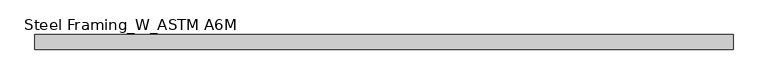
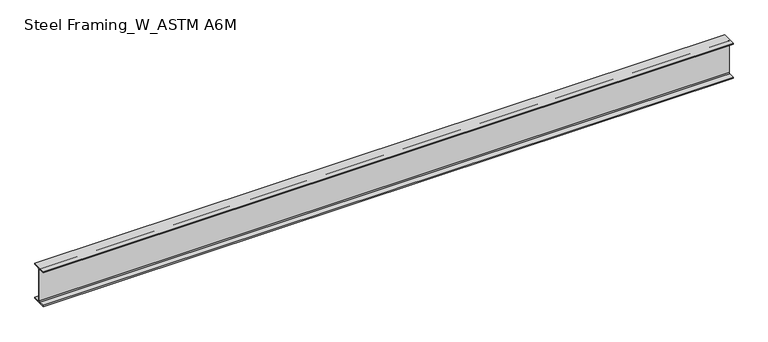
"""IFC4 building model written with IfcOpenShell, lengths in millimetres: beam geometry, Steel Framing_W_ASTM A6M : H_SB_AR_S02_W530x101_RB1."""

from ifc_helpers import new_model, si_unit, point, frame, frame_2d, origin, place, context, project, spatial, polyline, circle_curve, trimmed, segment, composite_curve, outline, extrude, source, transform, mapped, element, save


def steel_framing_w_astm_a6m_a5cbddeb(model_context):
    return source(origin(), model_context, "Body", "SweptSolid", [
        extrude(outline(composite_curve([segment(polyline([(105.0, -250.6), (105.0, -268.0), (-105.0, -268.0), (-105.0, -250.6), (-18.25, -250.6)]), True, "CONTINUOUS"), segment(trimmed(circle_curve(frame_2d((-18.25, -237.8)), 12.8), [point((-18.25, -250.6))], [point((-5.45, -237.8))], True, "CARTESIAN"), True, "CONTINUOUS"), segment(polyline([(-5.45, -237.8), (-5.45, 237.8)]), True, "CONTINUOUS"), segment(trimmed(circle_curve(frame_2d((-18.25, 237.8)), 12.8), [point((-5.45, 237.8))], [point((-18.25, 250.6))], True, "CARTESIAN"), True, "CONTINUOUS"), segment(polyline([(-18.25, 250.6), (-105.0, 250.6), (-105.0, 268.0), (105.0, 268.0), (105.0, 250.6), (18.25, 250.6)]), True, "CONTINUOUS"), segment(trimmed(circle_curve(frame_2d((18.25, 237.8)), 12.8), [point((18.25, 250.6))], [point((5.45, 237.8))], True, "CARTESIAN"), True, "CONTINUOUS"), segment(polyline([(5.45, 237.8), (5.45, -237.8)]), True, "CONTINUOUS"), segment(trimmed(circle_curve(frame_2d((18.25, -237.8)), 12.8), [point((5.45, -237.8))], [point((18.25, -250.6))], True, "CARTESIAN"), True, "CONTINUOUS"), segment(polyline([(18.25, -250.6), (105.0, -250.6)]), True, "CONTINUOUS")], self_intersect=False)), frame((-5000.0, 0.0, 0.0), z_axis=(1.0, 0.0, 0.0), x_axis=(0.0, 1.0, 0.0)), (0.0, 0.0, 1.0), 10000.0),
    ])


if __name__ == "__main__":
    model = new_model("IFC4")
    model_context = context("Model", 3, world=origin())
    ifc_project = project(units=[si_unit("LENGTHUNIT", "METRE", prefix="MILLI")], contexts=[model_context])
    site = spatial("IfcSite", under=ifc_project)
    building = spatial("IfcBuilding", under=site)
    placement = place(None, origin())
    steel_framing_w_astm_a6m_shape = steel_framing_w_astm_a6m_a5cbddeb(model_context)
    element("IfcBeam", 1, ObjectType="Steel Framing_W_ASTM A6M : H_SB_AR_S02_W530x101_RB1", at=placement, inside=building, context=model_context, shape_type="MappedRepresentation", body=[
        mapped(steel_framing_w_astm_a6m_shape, transform((0.0, 0.0, 0.0), x_axis=(1.0, 0.0, 0.0), y_axis=(0.0, 1.0, 0.0), z_axis=(0.0, 0.0, 1.0))),
    ])
    save(model, "model.ifc")

# Revit data of these elements
# Type "Steel Framing_W_ASTM A6M : H_SB_AR_S02_W530x101_RB1"
#   Type Mark = "RB1"
#   Section Name Key = "W21x68"
#   Width = 21.0 cm
#   Web Thickness = 1.09 cm
#   Web Fillet = 1.28 cm
#   Warping Constant = 1820000.0 cm⁶
#   Torsional Moment of Inertia = 102.00 cm⁴
#   Section Area = 129.0 cm²
#   Plastic Modulus weak axis = 400.0 cm³
#   Plastic Modulus strong axis = 2620.0 cm³
#   Perimeter = 1.87 m²/m
#   Nominal Weight = 101.00 kgf/m
#   Moment of Inertia weak axis = 2690.00 cm⁴
#   Moment of Inertia strong axis = 61600.00 cm⁴
#   Height = 53.6 cm
#   Flange Thickness = 1.74 cm
#   Elastic Modulus weak axis = 257.0 cm³
#   Elastic Modulus strong axis = 2290.0 cm³
#   Centroid Vertical = 26.8 cm
#   Centroid Horizontal = 10.5 cm
#   Length [instance default] = 1500 mm
#   Structural Material [instance default] = Steel, 45-345
#   Bolt Spacing = 0
#   Assembly Code = ""
# Element 1 (IfcBeam, "Steel Framing_W_ASTM A6M : H_SB_AR_S02_W530x101_RB1")
#   Materials on its faces: "Steel, 45-345"
# Materials
#   "Steel, 45-345": class "Metal", colour RGB 189 187 185, transparency 0, Description = "Steel 345 MPa", Cost = 0
